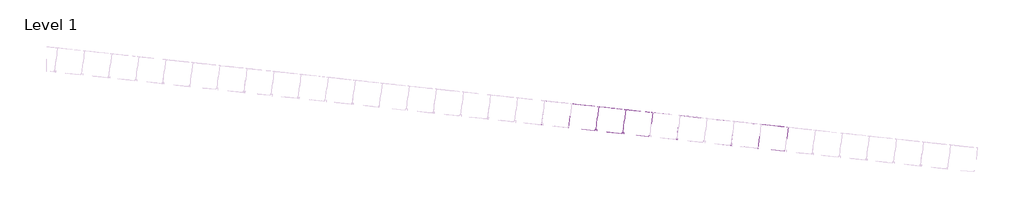
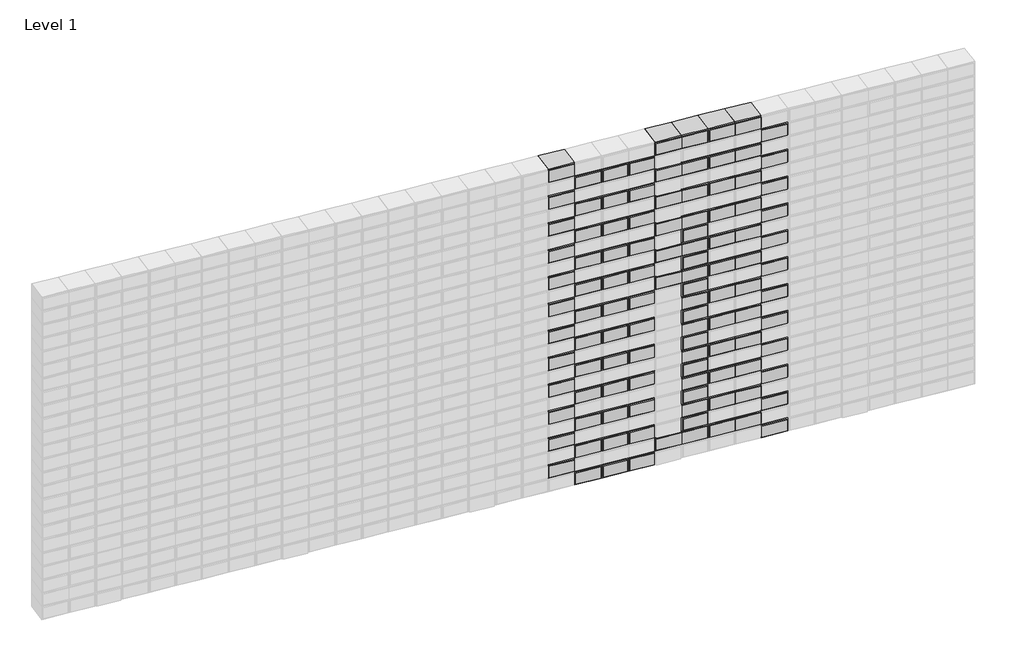
# One storey, part 16 of 18: 111 proxies.
# Revit data of these elements (continued)
# Elements 56, 57, 58, 59, 60, 61, 62, 63, 64, 65, 66, 67, 68, 69, 70, 71, 72, 73, 74, 75, 76, 77, 78, 79 (IfcBuildingElementProxy, "00_GMA_steen_versie_6 : Rood") (continued)
#   Materials on its faces: "20_voeg", "21_steen_rood"
# Elements 80, 81, 82, 83, 84, 85, 86, 87, 88, 89, 90, 91, 92, 93, 94, 95, 96, 97, 98, 99, 100, 101, 102, 103, 104, 105, 106, 107, 108, 109, 110, 111 (IfcBuildingElementProxy, "00_GMA_steen_versie_6 : Rood")
#   StootvoegLinksHalfOnder = 5 mm
#   StootvoegLinksHalfBoven = 5 mm
#   StootVoegRechtsHalfOnder = 5 mm
#   StootVoegRechtsHalfBoven = 5 mm
#   StootVoegBreedteRechts = 10 mm
#   StootVoegBreedteLinks = 10 mm
#   LintVoegOnderHalf = 5 mm
#   LintVoegOnder = 10 mm
#   LintVoegBovenHalf = 5 mm
#   LintVoegBoven = 10 mm
#   Phase Created = New Construction
#   Materials on its faces: "20_voeg", "21_steen_rood"
# Materials
#   "21_steen_geel": class "Unassigned", colour RGB 202 202 0, transparency 0, Cost = 0
#   "20_voeg": class "Concrete", colour RGB 86 86 86, transparency 0, Manufacturer = "RevitGG", URL = "www.revitgg.nl", Description = "zandcement, generiek materiaal", Cost = 0
#   "21_steen_rood": class "Unassigned", colour RGB 213 111 43, transparency 0, Cost = 0
